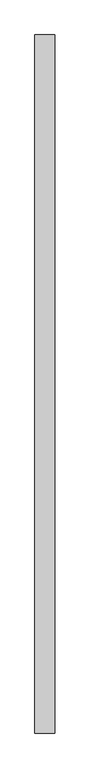
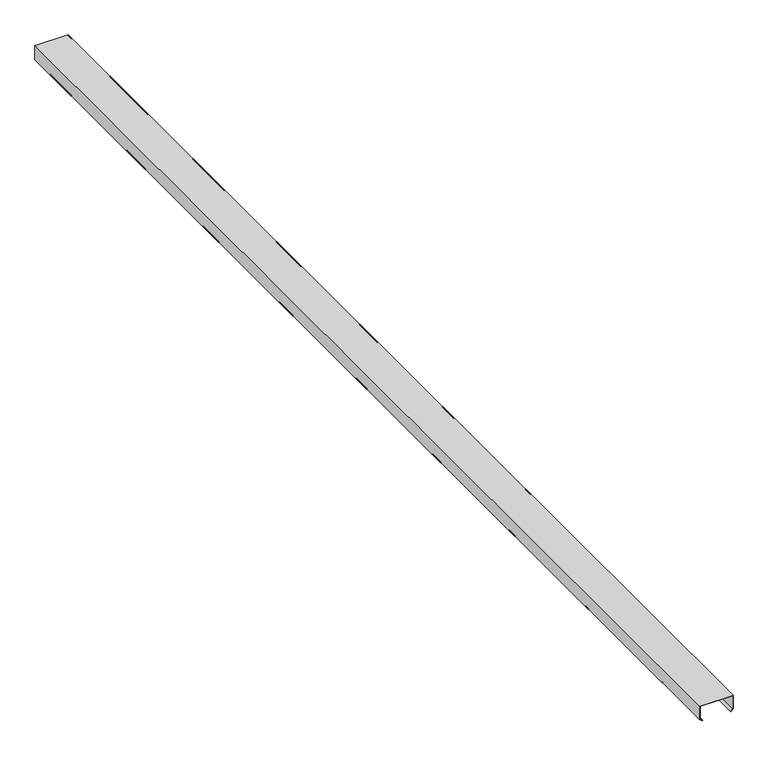
"""IFC4 building model written with IfcOpenShell, lengths in millimetres: proxy geometry, Generic Models 7:Generic Models 1:1:Generic Models 1:1 : Generic Models 7:Generic Models 1:337419:26 : Generic Models 7:Generic Models 1:1:Generic Models 1:1 : Generic Models 7:Generic Models 1:337419:306201."""

from ifc_helpers import new_model, si_unit, frame, origin, place, context, project, spatial, polyline, outline, extrude, source, transform, mapped, element, save


def generic_models_9008d6e7(model_context):
    return source(origin(), model_context, "Body", "SweptSolid", [
        extrude(outline(polyline([(4243.1890625, 560556.1617239), (4243.1890625, 560352.9617239), (4154.2890625, 560352.9617239), (4142.0439586, 560367.5548705), (4144.1721258, 560369.3406148), (4155.5845235, 560355.7398489), (4240.4109375, 560355.7398489), (4240.4109375, 560553.3835989), (4155.5845235, 560553.3835989), (4144.1721258, 560539.7828329), (4142.0439586, 560541.5685772), (4154.2890625, 560556.1617239), (4243.1890625, 560556.1617239)])), frame((0.0, -578752.4153396, 0.0), z_axis=(0.0, 1.0, 0.0), x_axis=(0.0, 0.0, 1.0)), (0.0, 0.0, 1.0), 7066.9239556),
    ])


if __name__ == "__main__":
    model = new_model("IFC4")
    model_context = context("Model", 3, world=origin())
    ifc_project = project(units=[si_unit("LENGTHUNIT", "METRE", prefix="MILLI")], contexts=[model_context])
    site = spatial("IfcSite", under=ifc_project)
    building = spatial("IfcBuilding", under=site)
    placement = place(None, origin())
    generic_models_shape = generic_models_9008d6e7(model_context)
    element("IfcBuildingElementProxy", 1, Name="Generic Models 7:Generic Models 1:1:Generic Models 1:1 : Generic Models 7:Generic Models 1:337419:26 : Generic Models 7:Generic Models 1:1:Generic Models 1:1 : Generic Models 7:Generic Models 1:337419:306201", ObjectType="Generic Models 7:Generic Models 1:1:Generic Models 1:1 : Generic Models 7:Generic Models 1:337419:26 : Generic Models 7:Generic Models 1:1:Generic Models 1:1 : Generic Models 7:Generic Models 1:337419:306201", at=placement, inside=building, context=model_context, shape_type="MappedRepresentation", body=[
        mapped(generic_models_shape, transform((0.0, 0.0, 0.0), x_axis=(1.0, 0.0, 0.0), y_axis=(0.0, 1.0, 0.0), z_axis=(0.0, 0.0, 1.0))),
    ])
    save(model, "model.ifc")

# Revit data of these elements
# Type "Generic Models 7:Generic Models 1:1:Generic Models 1:1 : Generic Models 7:Generic Models 1:337419:26 : Generic Models 7:Generic Models 1:1:Generic Models 1:1 : Generic Models 7:Generic Models 1:337419:306201"
#   NameOverride = "Generic Models 7:Generic Models 1:1:Generic Models 1:1 : Generic Models 7:Generic Models 1:337419:306201"
#   ObjectTypeOverride = "Generic Models 1:1 : Generic Models 7:Generic Models 1:337419"
#   Reference = "Generic Models 1"
#   Tag = "306201"
# Element 1 (IfcBuildingElementProxy, "Generic Models 7:Generic Models 1:1:Generic Models 1:1 : Generic Models 7:Generic Models 1:337419:26 : Generic Models 7:Generic Models 1:1:Generic Models 1:1 : Generic Models 7:Generic Models 1:337419:306201")
#   Materials on its faces: "GALVANIZED 'CEE' SECTION (8.0x3.5C - SEE STRUCT. DWGS)"
# Materials
#   "GALVANIZED 'CEE' SECTION (8.0x3.5C - SEE STRUCT. DWGS)": class "Unassigned", colour RGB 210 209 208, transparency 0, Keynote = "M05121300.02", Cost = 0
